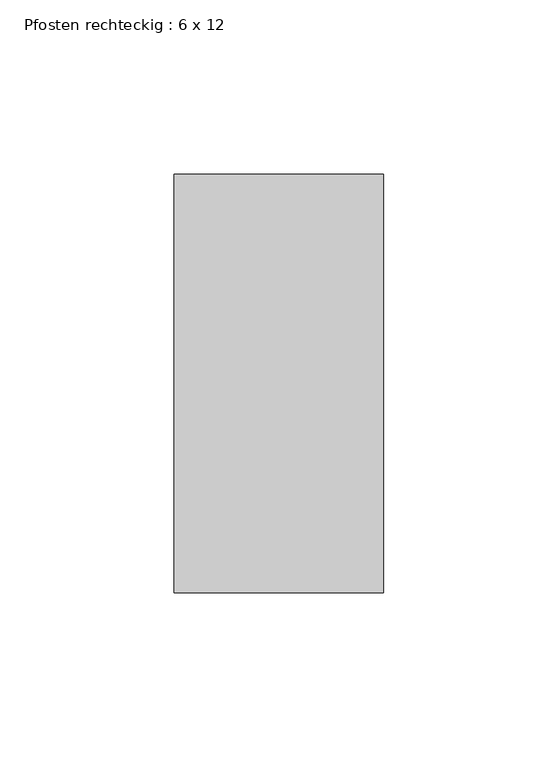
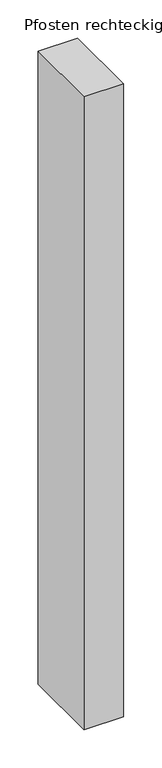
"""IFC4 building model written with IfcOpenShell, lengths in millimetres: member geometry, Pfosten rechteckig : 6 x 12."""

from ifc_helpers import new_model, si_unit, frame, origin, place, context, project, spatial, polyline, outline, extrude, source, transform, mapped, element, save


def pfosten_rechteckig_6_x_12_fe322a11(model_context):
    return source(origin(), model_context, "Body", "SweptSolid", [
        extrude(outline(polyline([(0.0, 60.0), (0.0, -60.0), (-60.0, -60.0), (-60.0, 60.0), (0.0, 60.0)])), frame((0.0, 0.0, -1009.9773049), z_axis=(0.0, 0.0, 1.0), x_axis=(1.0, 0.0, 0.0)), (0.0, 0.0, 1.0), 1009.9773049),
    ])


if __name__ == "__main__":
    model = new_model("IFC4")
    model_context = context("Model", 3, world=origin())
    ifc_project = project(units=[si_unit("LENGTHUNIT", "METRE", prefix="MILLI")], contexts=[model_context])
    site = spatial("IfcSite", under=ifc_project)
    building = spatial("IfcBuilding", under=site)
    placement = place(None, origin())
    pfosten_rechteckig_6_x_12_shape = pfosten_rechteckig_6_x_12_fe322a11(model_context)
    element("IfcMember", 1, ObjectType="Pfosten rechteckig : 6 x 12", at=placement, inside=building, context=model_context, shape_type="MappedRepresentation", body=[
        mapped(pfosten_rechteckig_6_x_12_shape, transform((0.0, 0.0, 0.0), x_axis=(1.0, 0.0, 0.0), y_axis=(0.0, 1.0, 0.0), z_axis=(0.0, 0.0, 1.0))),
    ])
    save(model, "model.ifc")

# Revit data of these elements
# Type "Pfosten rechteckig : 6 x 12"
#   built-in parameter 1007304 = 0.393701 (stored number, unit not read)
#   built-in parameter 1007301 = 0.0984252 (stored number, unit not read)
#   built-in parameter 1007300 = 0.0984252 (stored number, unit not read)
# Element 1 (IfcMember, "Pfosten rechteckig : 6 x 12")
#   Materials on its faces: "Metall - verzinkt"
# Materials
#   "Metall - verzinkt": class "Allgemeines", colour RGB 200 200 200, transparency 0, Cost = 0
